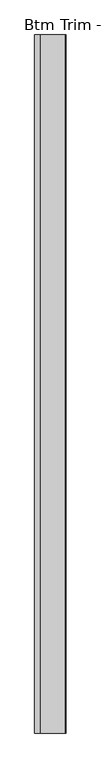
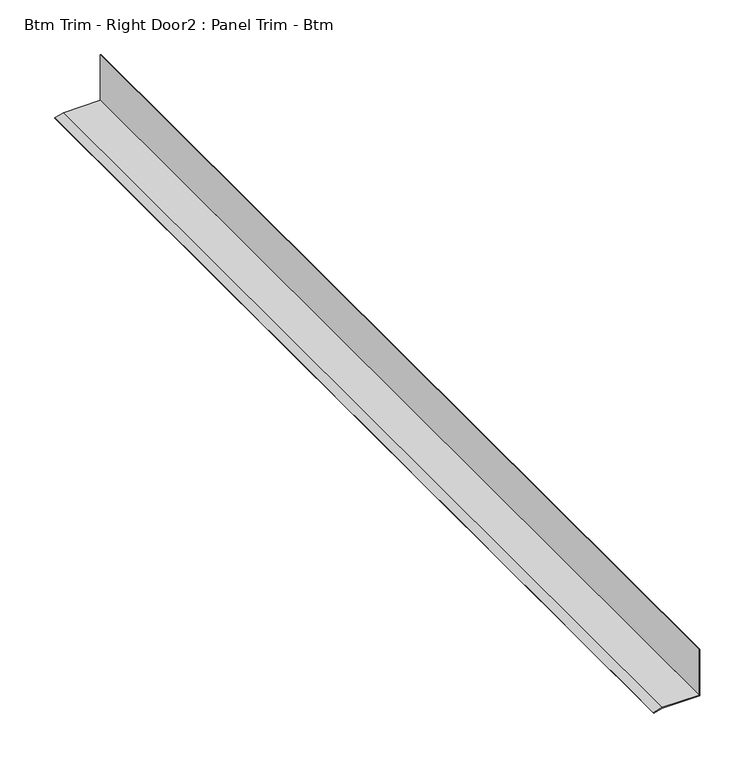
"""IFC4 building model written with IfcOpenShell, lengths in millimetres: proxy geometry, Btm Trim - Right Door2 : Panel Trim - Btm."""

import ifcopenshell
import ifcopenshell.guid

model = None  # the IFC model being written
_history = None  # IfcOwnerHistory: only IFC2X3 demands one
_inside = {}  # id of a spatial element -> (the spatial element, [elements in it])
_under = {}  # id of a project, library or spatial element -> (it, [spatial elements below it])
_declared = {}  # id of a project -> (the project, [libraries it declares])
_typed = {}  # id of a type object -> (the type object, [elements of that type])
_made_of = {}  # id of a material, layer set ... -> (it, [elements and type objects made of it])


def new_model(schema):
    """Start an empty IFC model of exactly this schema.

    Asked for "IFC4X3", IfcOpenShell would pick the latest addendum, in which some entities
    have other attributes; the version numbers below select the first issue.
    IFC2X3 requires an IfcOwnerHistory on every rooted entity: one is made here for all.
    """
    global model, _history
    if schema == "IFC4X3":
        model = ifcopenshell.file(schema_version=(4, 3, 0, 0))
    else:
        model = ifcopenshell.file(schema=schema)
    _inside.clear()
    _under.clear()
    _declared.clear()
    _typed.clear()
    _made_of.clear()
    _history = None
    if model.schema == "IFC2X3":
        org = make("IfcOrganization", Name="unknown")
        user = make(
            "IfcPersonAndOrganization",
            ThePerson=make("IfcPerson", FamilyName="unknown"),
            TheOrganization=org,
        )
        app = make(
            "IfcApplication",
            ApplicationDeveloper=org,
            Version="unknown",
            ApplicationFullName="unknown",
            ApplicationIdentifier="unknown",
        )
        _history = make(
            "IfcOwnerHistory",
            OwningUser=user,
            OwningApplication=app,
            ChangeAction="ADDED",
            CreationDate=0,
        )
    return model


def make(cls, **values):
    """One entity of the class cls with the attributes given. An attribute that is None is left unset."""
    return model.create_entity(
        cls, **{name: value for name, value in values.items() if value is not None}
    )


def rooted(cls, **values):
    """An entity with a GlobalId (a new one), such as an element, a storey or a relation."""
    return make(cls, GlobalId=ifcopenshell.guid.new(), OwnerHistory=_history, **values)


def si_unit(unit_type, name, prefix=None):
    """IfcSIUnit, for example si_unit("LENGTHUNIT", "METRE", prefix="MILLI")."""
    return make("IfcSIUnit", UnitType=unit_type, Prefix=prefix, Name=name)


def assignment(units):
    """IfcUnitAssignment: the units of a project."""
    return None if units is None else make("IfcUnitAssignment", Units=units)


def point(xyz):
    """IfcCartesianPoint."""
    return None if xyz is None else make("IfcCartesianPoint", Coordinates=xyz)


def direction(xyz):
    """IfcDirection."""
    return None if xyz is None else make("IfcDirection", DirectionRatios=xyz)


def frame(location, z_axis=None, x_axis=None):
    """IfcAxis2Placement3D, a coordinate frame: its origin and axes. An axis left out is left unset."""
    return make(
        "IfcAxis2Placement3D",
        Location=point(location),
        Axis=direction(z_axis),
        RefDirection=direction(x_axis),
    )


def origin():
    """The frame at (0, 0, 0) with its axes left unset."""
    return frame((0.0, 0.0, 0.0))


def place(relative_to, where):
    """IfcLocalPlacement: puts the frame where relative to a parent placement (None: the world)."""
    return make(
        "IfcLocalPlacement", PlacementRelTo=relative_to, RelativePlacement=where
    )


def context(
    kind, dimensions, precision=None, world=None, true_north=None, identifier=None
):
    """IfcGeometricRepresentationContext, for example the 3D "Model" context."""
    return make(
        "IfcGeometricRepresentationContext",
        ContextIdentifier=identifier,
        ContextType=kind,
        CoordinateSpaceDimension=dimensions,
        Precision=precision,
        WorldCoordinateSystem=world,
        TrueNorth=true_north,
    )


def project(units=None, contexts=None):
    """IfcProject with its units and contexts."""
    return rooted(
        "IfcProject",
        Name="project",
        RepresentationContexts=contexts,
        UnitsInContext=assignment(units),
    )


def spatial(cls, under=None, at=None, **own):
    """A site, building, storey or space (cls), placed at a placement, below another one or the project."""
    s = rooted(cls, ObjectPlacement=at, **own)
    if under is not None:
        _under.setdefault(under.id(), (under, []))[1].append(s)
    return s


def polyline(points):
    """IfcPolyline through the points."""
    return make("IfcPolyline", Points=[point(p) for p in points])


def outline(outer, holes=None, kind="AREA"):
    """IfcArbitraryClosedProfileDef: a profile drawn as a closed curve; with holes, ...WithVoids."""
    if holes is None:
        return make("IfcArbitraryClosedProfileDef", ProfileType=kind, OuterCurve=outer)
    return make(
        "IfcArbitraryProfileDefWithVoids",
        ProfileType=kind,
        OuterCurve=outer,
        InnerCurves=holes,
    )


def extrude(swept, where, along, depth):
    """IfcExtrudedAreaSolid: the profile swept, set in the frame where, extruded along a direction by depth."""
    return make(
        "IfcExtrudedAreaSolid",
        SweptArea=swept,
        Position=where,
        ExtrudedDirection=direction(along),
        Depth=depth,
    )


def shape(context_of_items, identifier, shape_type, items):
    """IfcShapeRepresentation: the items that make up one representation, for example the "Body"."""
    return make(
        "IfcShapeRepresentation",
        ContextOfItems=context_of_items,
        RepresentationIdentifier=identifier,
        RepresentationType=shape_type,
        Items=items,
    )


def source(mapping_origin, context_of_items, identifier, shape_type, items):
    """IfcRepresentationMap: a shape defined once, which mapped items show again and again."""
    return make(
        "IfcRepresentationMap",
        MappingOrigin=mapping_origin,
        MappedRepresentation=shape(context_of_items, identifier, shape_type, items),
    )


def transform(
    local_origin,
    x_axis=None,
    y_axis=None,
    z_axis=None,
    scale=None,
    scale2=None,
    scale3=None,
    uniform=True,
):
    """IfcCartesianTransformationOperator3D, or its non-uniform kind. x_axis, y_axis, z_axis: its Axis1, 2, 3."""
    if uniform:
        return make(
            "IfcCartesianTransformationOperator3D",
            Axis1=direction(x_axis),
            Axis2=direction(y_axis),
            LocalOrigin=point(local_origin),
            Scale=scale,
            Axis3=direction(z_axis),
        )
    return make(
        "IfcCartesianTransformationOperator3DnonUniform",
        Axis1=direction(x_axis),
        Axis2=direction(y_axis),
        LocalOrigin=point(local_origin),
        Scale=scale,
        Axis3=direction(z_axis),
        Scale2=scale2,
        Scale3=scale3,
    )


def mapped(mapping_source, mapping_target):
    """IfcMappedItem: shows the shape of a source again, moved by a transform."""
    return make(
        "IfcMappedItem", MappingSource=mapping_source, MappingTarget=mapping_target
    )


def made_of(thing, what):
    """Note that an element or type object is made of a material, layer set ...; save() writes the relation."""
    if what is not None:
        _made_of.setdefault(what.id(), (what, []))[1].append(thing)
    return thing


def element(
    cls,
    number,
    at=None,
    inside=None,
    cuts=None,
    type_object=None,
    material=None,
    context=None,
    identifier="Body",
    shape_type=None,
    held_by="IfcProductDefinitionShape",
    body=None,
    shapes=None,
    **own,
):
    """One element of the class cls, such as IfcWall. Its Tag is "e" and its number.

    at: its placement. inside: the storey or other place that contains it. cuts: it is an
    opening in that element (IfcRelVoidsElement). A single representation is given by context,
    identifier, shape_type and body (its items); several are given by shapes. held_by: the class
    of the entity that holds the representations. save() writes the other relations.
    """
    e = rooted(cls, Tag="e%d" % number, ObjectPlacement=at, **own)
    if body is not None:
        shapes = [shape(context, identifier, shape_type, body)]
    if shapes is not None:
        e.Representation = make(held_by, Representations=shapes)
    if inside is not None:
        _inside.setdefault(inside.id(), (inside, []))[1].append(e)
    if cuts is not None:
        rooted(
            "IfcRelVoidsElement", RelatingBuildingElement=cuts, RelatedOpeningElement=e
        )
    if type_object is not None:
        _typed.setdefault(type_object.id(), (type_object, []))[1].append(e)
    return made_of(e, material)


def aggregate(whole, parts):
    """IfcRelAggregates: a whole, such as a stair, and the parts it consists of."""
    return rooted("IfcRelAggregates", RelatingObject=whole, RelatedObjects=parts)


def save(model, path):
    """Write the relations noted so far, then the file.

    IfcRelAggregates (storeys below a building ...), IfcRelContainedInSpatialStructure (elements
    in a storey), IfcRelDefinesByType, IfcRelAssociatesMaterial and IfcRelDeclares: one each for
    every whole, place, type object, material and project.
    """
    for whole, parts in _under.values():
        aggregate(whole, parts)
    for where, things in _inside.values():
        rooted(
            "IfcRelContainedInSpatialStructure",
            RelatedElements=things,
            RelatingStructure=where,
        )
    for kind, things in _typed.values():
        rooted("IfcRelDefinesByType", RelatedObjects=things, RelatingType=kind)
    for what, things in _made_of.values():
        rooted("IfcRelAssociatesMaterial", RelatedObjects=things, RelatingMaterial=what)
    for by, libraries in _declared.values():
        rooted("IfcRelDeclares", RelatingContext=by, RelatedDefinitions=libraries)
    model.write(path)


def btm_trim_right_door2_panel_trim_btm_5f1d7bb7(model_context):
    return source(origin(), model_context, "Body", "SweptSolid", [
        extrude(outline(polyline([(50.8, 587326.1141748), (48.3077022, 587316.8127928), (47.5409986, 587317.0182304), (50.00625, 587326.2186739), (50.00625, 587365.8934739), (101.6, 587365.8934739), (101.6, 587365.1060739), (50.8, 587365.1060739), (50.8, 587326.1141748)])), frame((0.0, -533977.6038841, 0.0), z_axis=(0.0, 1.0, 0.0), x_axis=(0.0, 0.0, 1.0)), (0.0, 0.0, 1.0), 1094.5749),
    ])


if __name__ == "__main__":
    model = new_model("IFC4")
    model_context = context("Model", 3, world=origin())
    ifc_project = project(units=[si_unit("LENGTHUNIT", "METRE", prefix="MILLI")], contexts=[model_context])
    site = spatial("IfcSite", under=ifc_project)
    building = spatial("IfcBuilding", under=site)
    placement = place(None, origin())
    btm_trim_right_door2_panel_trim_btm_shape = btm_trim_right_door2_panel_trim_btm_5f1d7bb7(model_context)
    element("IfcBuildingElementProxy", 1, Name="Btm Trim - Right Door2 : Panel Trim - Btm", ObjectType="Btm Trim - Right Door2 : Panel Trim - Btm", at=placement, inside=building, context=model_context, shape_type="MappedRepresentation", body=[
        mapped(btm_trim_right_door2_panel_trim_btm_shape, transform((0.0, 0.0, 0.0), x_axis=(1.0, 0.0, 0.0), y_axis=(0.0, 1.0, 0.0), z_axis=(0.0, 0.0, 1.0))),
    ])
    save(model, "model.ifc")

# Revit data of these elements
# Element 1 (IfcBuildingElementProxy, "Btm Trim - Right Door2 : Panel Trim - Btm")
#   Materials on its faces: "BASE TRIM BY MTL PANEL MFR."
# Materials
#   "BASE TRIM BY MTL PANEL MFR.": class "Generic", colour RGB 239 242 240, transparency 0, Cost = 0
